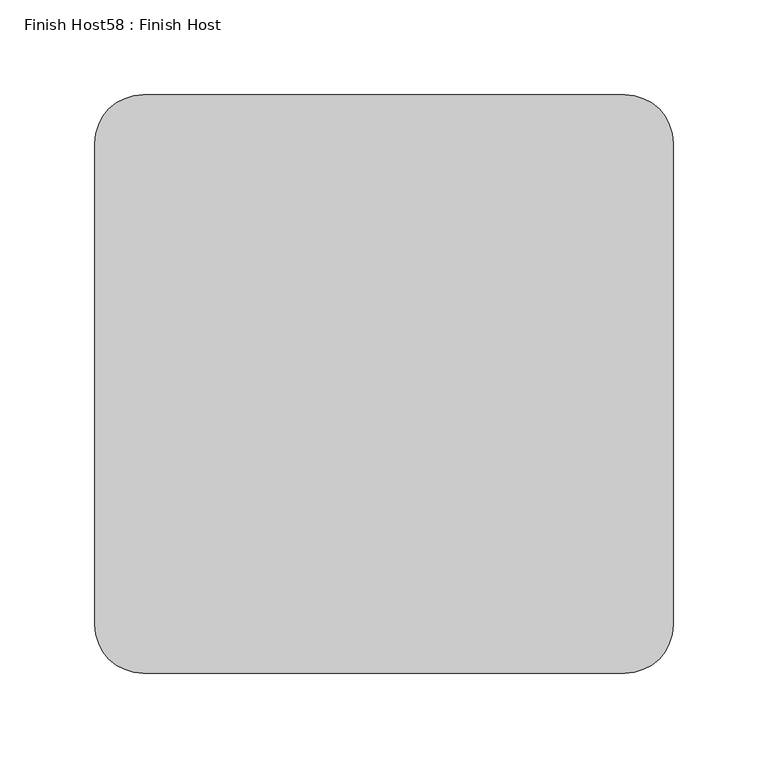
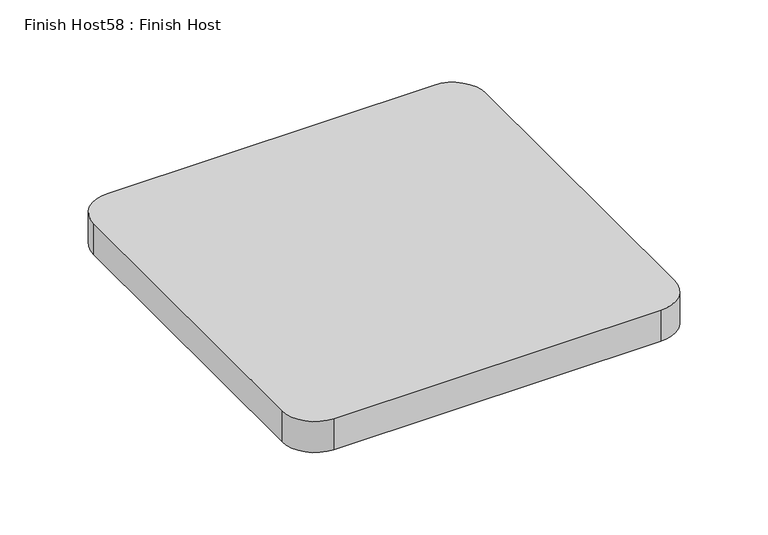
"""IFC4 building model written with IfcOpenShell, lengths in millimetres: proxy geometry, Finish Host58 : Finish Host."""

import ifcopenshell
import ifcopenshell.guid

model = None  # the IFC model being written
_history = None  # IfcOwnerHistory: only IFC2X3 demands one
_inside = {}  # id of a spatial element -> (the spatial element, [elements in it])
_under = {}  # id of a project, library or spatial element -> (it, [spatial elements below it])
_declared = {}  # id of a project -> (the project, [libraries it declares])
_typed = {}  # id of a type object -> (the type object, [elements of that type])
_made_of = {}  # id of a material, layer set ... -> (it, [elements and type objects made of it])


def new_model(schema):
    """Start an empty IFC model of exactly this schema.

    Asked for "IFC4X3", IfcOpenShell would pick the latest addendum, in which some entities
    have other attributes; the version numbers below select the first issue.
    IFC2X3 requires an IfcOwnerHistory on every rooted entity: one is made here for all.
    """
    global model, _history
    if schema == "IFC4X3":
        model = ifcopenshell.file(schema_version=(4, 3, 0, 0))
    else:
        model = ifcopenshell.file(schema=schema)
    _inside.clear()
    _under.clear()
    _declared.clear()
    _typed.clear()
    _made_of.clear()
    _history = None
    if model.schema == "IFC2X3":
        org = make("IfcOrganization", Name="unknown")
        user = make(
            "IfcPersonAndOrganization",
            ThePerson=make("IfcPerson", FamilyName="unknown"),
            TheOrganization=org,
        )
        app = make(
            "IfcApplication",
            ApplicationDeveloper=org,
            Version="unknown",
            ApplicationFullName="unknown",
            ApplicationIdentifier="unknown",
        )
        _history = make(
            "IfcOwnerHistory",
            OwningUser=user,
            OwningApplication=app,
            ChangeAction="ADDED",
            CreationDate=0,
        )
    return model


def make(cls, **values):
    """One entity of the class cls with the attributes given. An attribute that is None is left unset."""
    return model.create_entity(
        cls, **{name: value for name, value in values.items() if value is not None}
    )


def rooted(cls, **values):
    """An entity with a GlobalId (a new one), such as an element, a storey or a relation."""
    return make(cls, GlobalId=ifcopenshell.guid.new(), OwnerHistory=_history, **values)


def si_unit(unit_type, name, prefix=None):
    """IfcSIUnit, for example si_unit("LENGTHUNIT", "METRE", prefix="MILLI")."""
    return make("IfcSIUnit", UnitType=unit_type, Prefix=prefix, Name=name)


def assignment(units):
    """IfcUnitAssignment: the units of a project."""
    return None if units is None else make("IfcUnitAssignment", Units=units)


def point(xyz):
    """IfcCartesianPoint."""
    return None if xyz is None else make("IfcCartesianPoint", Coordinates=xyz)


def direction(xyz):
    """IfcDirection."""
    return None if xyz is None else make("IfcDirection", DirectionRatios=xyz)


def frame(location, z_axis=None, x_axis=None):
    """IfcAxis2Placement3D, a coordinate frame: its origin and axes. An axis left out is left unset."""
    return make(
        "IfcAxis2Placement3D",
        Location=point(location),
        Axis=direction(z_axis),
        RefDirection=direction(x_axis),
    )


def frame_2d(location, x_axis=None):
    """IfcAxis2Placement2D, a coordinate frame in the plane: its origin and x axis."""
    return make(
        "IfcAxis2Placement2D", Location=point(location), RefDirection=direction(x_axis)
    )


def origin():
    """The frame at (0, 0, 0) with its axes left unset."""
    return frame((0.0, 0.0, 0.0))


def origin_with_axes():
    """The frame at (0, 0, 0) with the z axis (0, 0, 1) and the x axis (1, 0, 0) written out."""
    return frame((0.0, 0.0, 0.0), z_axis=(0.0, 0.0, 1.0), x_axis=(1.0, 0.0, 0.0))


def place(relative_to, where):
    """IfcLocalPlacement: puts the frame where relative to a parent placement (None: the world)."""
    return make(
        "IfcLocalPlacement", PlacementRelTo=relative_to, RelativePlacement=where
    )


def context(
    kind, dimensions, precision=None, world=None, true_north=None, identifier=None
):
    """IfcGeometricRepresentationContext, for example the 3D "Model" context."""
    return make(
        "IfcGeometricRepresentationContext",
        ContextIdentifier=identifier,
        ContextType=kind,
        CoordinateSpaceDimension=dimensions,
        Precision=precision,
        WorldCoordinateSystem=world,
        TrueNorth=true_north,
    )


def project(units=None, contexts=None):
    """IfcProject with its units and contexts."""
    return rooted(
        "IfcProject",
        Name="project",
        RepresentationContexts=contexts,
        UnitsInContext=assignment(units),
    )


def spatial(cls, under=None, at=None, **own):
    """A site, building, storey or space (cls), placed at a placement, below another one or the project."""
    s = rooted(cls, ObjectPlacement=at, **own)
    if under is not None:
        _under.setdefault(under.id(), (under, []))[1].append(s)
    return s


def polyline(points):
    """IfcPolyline through the points."""
    return make("IfcPolyline", Points=[point(p) for p in points])


def circle_curve(where, radius):
    """IfcCircle in the frame where."""
    return make("IfcCircle", Position=where, Radius=radius)


def trimmed(basis, trim1, trim2, sense, master):
    """IfcTrimmedCurve: the piece of a basis curve between two trims."""
    return make(
        "IfcTrimmedCurve",
        BasisCurve=basis,
        Trim1=trim1,
        Trim2=trim2,
        SenseAgreement=sense,
        MasterRepresentation=master,
    )


def segment(curve, same_sense, transition):
    """IfcCompositeCurveSegment."""
    return make(
        "IfcCompositeCurveSegment",
        Transition=transition,
        SameSense=same_sense,
        ParentCurve=curve,
    )


def composite_curve(segments, self_intersect=None):
    """IfcCompositeCurve: segments joined end to end."""
    return make("IfcCompositeCurve", Segments=segments, SelfIntersect=self_intersect)


def outline(outer, holes=None, kind="AREA"):
    """IfcArbitraryClosedProfileDef: a profile drawn as a closed curve; with holes, ...WithVoids."""
    if holes is None:
        return make("IfcArbitraryClosedProfileDef", ProfileType=kind, OuterCurve=outer)
    return make(
        "IfcArbitraryProfileDefWithVoids",
        ProfileType=kind,
        OuterCurve=outer,
        InnerCurves=holes,
    )


def extrude(swept, where, along, depth):
    """IfcExtrudedAreaSolid: the profile swept, set in the frame where, extruded along a direction by depth."""
    return make(
        "IfcExtrudedAreaSolid",
        SweptArea=swept,
        Position=where,
        ExtrudedDirection=direction(along),
        Depth=depth,
    )


def shape(context_of_items, identifier, shape_type, items):
    """IfcShapeRepresentation: the items that make up one representation, for example the "Body"."""
    return make(
        "IfcShapeRepresentation",
        ContextOfItems=context_of_items,
        RepresentationIdentifier=identifier,
        RepresentationType=shape_type,
        Items=items,
    )


def source(mapping_origin, context_of_items, identifier, shape_type, items):
    """IfcRepresentationMap: a shape defined once, which mapped items show again and again."""
    return make(
        "IfcRepresentationMap",
        MappingOrigin=mapping_origin,
        MappedRepresentation=shape(context_of_items, identifier, shape_type, items),
    )


def transform(
    local_origin,
    x_axis=None,
    y_axis=None,
    z_axis=None,
    scale=None,
    scale2=None,
    scale3=None,
    uniform=True,
):
    """IfcCartesianTransformationOperator3D, or its non-uniform kind. x_axis, y_axis, z_axis: its Axis1, 2, 3."""
    if uniform:
        return make(
            "IfcCartesianTransformationOperator3D",
            Axis1=direction(x_axis),
            Axis2=direction(y_axis),
            LocalOrigin=point(local_origin),
            Scale=scale,
            Axis3=direction(z_axis),
        )
    return make(
        "IfcCartesianTransformationOperator3DnonUniform",
        Axis1=direction(x_axis),
        Axis2=direction(y_axis),
        LocalOrigin=point(local_origin),
        Scale=scale,
        Axis3=direction(z_axis),
        Scale2=scale2,
        Scale3=scale3,
    )


def mapped(mapping_source, mapping_target):
    """IfcMappedItem: shows the shape of a source again, moved by a transform."""
    return make(
        "IfcMappedItem", MappingSource=mapping_source, MappingTarget=mapping_target
    )


def made_of(thing, what):
    """Note that an element or type object is made of a material, layer set ...; save() writes the relation."""
    if what is not None:
        _made_of.setdefault(what.id(), (what, []))[1].append(thing)
    return thing


def element(
    cls,
    number,
    at=None,
    inside=None,
    cuts=None,
    type_object=None,
    material=None,
    context=None,
    identifier="Body",
    shape_type=None,
    held_by="IfcProductDefinitionShape",
    body=None,
    shapes=None,
    **own,
):
    """One element of the class cls, such as IfcWall. Its Tag is "e" and its number.

    at: its placement. inside: the storey or other place that contains it. cuts: it is an
    opening in that element (IfcRelVoidsElement). A single representation is given by context,
    identifier, shape_type and body (its items); several are given by shapes. held_by: the class
    of the entity that holds the representations. save() writes the other relations.
    """
    e = rooted(cls, Tag="e%d" % number, ObjectPlacement=at, **own)
    if body is not None:
        shapes = [shape(context, identifier, shape_type, body)]
    if shapes is not None:
        e.Representation = make(held_by, Representations=shapes)
    if inside is not None:
        _inside.setdefault(inside.id(), (inside, []))[1].append(e)
    if cuts is not None:
        rooted(
            "IfcRelVoidsElement", RelatingBuildingElement=cuts, RelatedOpeningElement=e
        )
    if type_object is not None:
        _typed.setdefault(type_object.id(), (type_object, []))[1].append(e)
    return made_of(e, material)


def aggregate(whole, parts):
    """IfcRelAggregates: a whole, such as a stair, and the parts it consists of."""
    return rooted("IfcRelAggregates", RelatingObject=whole, RelatedObjects=parts)


def save(model, path):
    """Write the relations noted so far, then the file.

    IfcRelAggregates (storeys below a building ...), IfcRelContainedInSpatialStructure (elements
    in a storey), IfcRelDefinesByType, IfcRelAssociatesMaterial and IfcRelDeclares: one each for
    every whole, place, type object, material and project.
    """
    for whole, parts in _under.values():
        aggregate(whole, parts)
    for where, things in _inside.values():
        rooted(
            "IfcRelContainedInSpatialStructure",
            RelatedElements=things,
            RelatingStructure=where,
        )
    for kind, things in _typed.values():
        rooted("IfcRelDefinesByType", RelatedObjects=things, RelatingType=kind)
    for what, things in _made_of.values():
        rooted("IfcRelAssociatesMaterial", RelatedObjects=things, RelatingMaterial=what)
    for by, libraries in _declared.values():
        rooted("IfcRelDeclares", RelatingContext=by, RelatedDefinitions=libraries)
    model.write(path)


def finish_host58_finish_host_489a3b4c(model_context):
    return source(origin(), model_context, "Body", "SweptSolid", [
        extrude(outline(composite_curve([segment(polyline([(-17113.2939795, 12994.4419385), (-17113.2939795, 13248.4419385)]), True, "CONTINUOUS"), segment(trimmed(circle_curve(frame_2d((-17087.8939795, 13248.4419385)), 25.4), [point((-17113.2939795, 13248.4419385))], [point((-17087.8939795, 13273.8419385))], False, "CARTESIAN"), True, "CONTINUOUS"), segment(polyline([(-17087.8939795, 13273.8419385), (-16833.8939795, 13273.8419385)]), True, "CONTINUOUS"), segment(trimmed(circle_curve(frame_2d((-16833.8939795, 13248.4419385)), 25.4), [point((-16833.8939795, 13273.8419385))], [point((-16808.4939795, 13248.4419385))], False, "CARTESIAN"), True, "CONTINUOUS"), segment(polyline([(-16808.4939795, 13248.4419385), (-16808.4939795, 12994.4419385)]), True, "CONTINUOUS"), segment(trimmed(circle_curve(frame_2d((-16833.8939795, 12994.4419385)), 25.4), [point((-16808.4939795, 12994.4419385))], [point((-16833.8939795, 12969.0419385))], False, "CARTESIAN"), True, "CONTINUOUS"), segment(polyline([(-16833.8939795, 12969.0419385), (-17087.8939795, 12969.0419385)]), True, "CONTINUOUS"), segment(trimmed(circle_curve(frame_2d((-17087.8939795, 12994.4419385)), 25.4), [point((-17087.8939795, 12969.0419385))], [point((-17113.2939795, 12994.4419385))], False, "CARTESIAN"), True, "CONTINUOUS")], self_intersect=False)), origin_with_axes(), (0.0, 0.0, 1.0), 25.4),
    ])


if __name__ == "__main__":
    model = new_model("IFC4")
    model_context = context("Model", 3, world=origin())
    ifc_project = project(units=[si_unit("LENGTHUNIT", "METRE", prefix="MILLI")], contexts=[model_context])
    site = spatial("IfcSite", under=ifc_project)
    building = spatial("IfcBuilding", under=site)
    placement = place(None, origin())
    finish_host58_finish_host_shape = finish_host58_finish_host_489a3b4c(model_context)
    element("IfcBuildingElementProxy", 1, Name="Finish Host58 : Finish Host", ObjectType="Finish Host58 : Finish Host", at=placement, inside=building, context=model_context, shape_type="MappedRepresentation", body=[
        mapped(finish_host58_finish_host_shape, transform((0.0, 0.0, 0.0), x_axis=(1.0, 0.0, 0.0), y_axis=(0.0, 1.0, 0.0), z_axis=(0.0, 0.0, 1.0))),
    ])
    save(model, "model.ifc")

# Revit data of these elements
# Type "Finish Host58 : Finish Host"
#   Panel Material = none
# Element 1 (IfcBuildingElementProxy, "Finish Host58 : Finish Host")
#   Materials on its faces: "Thread - Teknion - Sand"
# Materials
#   "Thread - Teknion - Sand": class "Fabric", colour RGB 138 122 89, transparency 0, Model = "F206", Manufacturer = "Teknion Studio", URL = "http://www.teknion.com/", Description = "Fantasme Full Wool", Cost = 0
